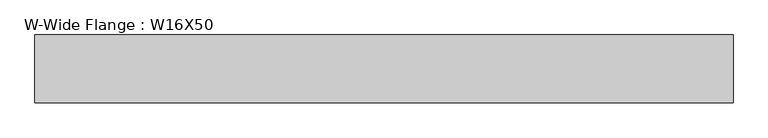
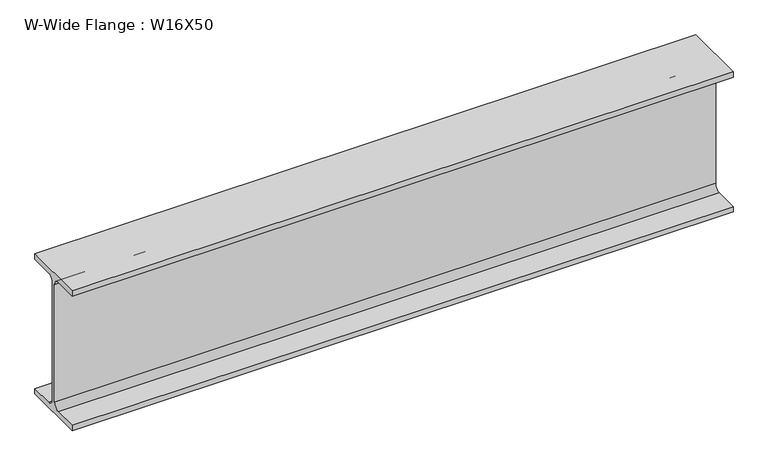
"""IFC4 building model written with IfcOpenShell, lengths in millimetres: beam geometry, W-Wide Flange : W16X50."""

from ifc_helpers import new_model, si_unit, point, frame, frame_2d, origin, place, context, project, spatial, polyline, circle_curve, trimmed, segment, composite_curve, outline, extrude, source, transform, mapped, element, save


def w_wide_flange_w16x50_f430b839(model_context):
    return source(origin(), model_context, "Body", "SweptSolid", [
        extrude(outline(composite_curve([segment(polyline([(-89.789, -191.008), (-22.1615, -191.008)]), True, "CONTINUOUS"), segment(trimmed(circle_curve(frame_2d((-22.1615, -173.6725)), 17.3355), [point((-22.1615, -191.008))], [point((-4.826, -173.6725))], True, "CARTESIAN"), True, "CONTINUOUS"), segment(polyline([(-4.826, -173.6725), (-4.826, 173.6725)]), True, "CONTINUOUS"), segment(trimmed(circle_curve(frame_2d((-22.1615, 173.6725)), 17.3355), [point((-4.826, 173.6725))], [point((-22.1615, 191.008))], True, "CARTESIAN"), True, "CONTINUOUS"), segment(polyline([(-22.1615, 191.008), (-89.789, 191.008), (-89.789, 207.01), (89.789, 207.01), (89.789, 191.008), (22.1615, 191.008)]), True, "CONTINUOUS"), segment(trimmed(circle_curve(frame_2d((22.1615, 173.6725)), 17.3355), [point((22.1615, 191.008))], [point((4.826, 173.6725))], True, "CARTESIAN"), True, "CONTINUOUS"), segment(polyline([(4.826, 173.6725), (4.826, -173.6725)]), True, "CONTINUOUS"), segment(trimmed(circle_curve(frame_2d((22.1615, -173.6725)), 17.3355), [point((4.826, -173.6725))], [point((22.1615, -191.008))], True, "CARTESIAN"), True, "CONTINUOUS"), segment(polyline([(22.1615, -191.008), (89.789, -191.008), (89.789, -207.01), (-89.789, -207.01), (-89.789, -191.008)]), True, "CONTINUOUS")], self_intersect=False)), frame((-912.045346, 0.0, 0.0), z_axis=(1.0, 0.0, 0.0), x_axis=(0.0, 1.0, 0.0)), (0.0, 0.0, 1.0), 1846.950692),
    ])


if __name__ == "__main__":
    model = new_model("IFC4")
    model_context = context("Model", 3, world=origin())
    ifc_project = project(units=[si_unit("LENGTHUNIT", "METRE", prefix="MILLI")], contexts=[model_context])
    site = spatial("IfcSite", under=ifc_project)
    building = spatial("IfcBuilding", under=site)
    placement = place(None, origin())
    w_wide_flange_w16x50_shape = w_wide_flange_w16x50_f430b839(model_context)
    element("IfcBeam", 1, ObjectType="W-Wide Flange : W16X50", at=placement, inside=building, context=model_context, shape_type="MappedRepresentation", body=[
        mapped(w_wide_flange_w16x50_shape, transform((0.0, 0.0, 0.0), x_axis=(1.0, 0.0, 0.0), y_axis=(0.0, 1.0, 0.0), z_axis=(0.0, 0.0, 1.0))),
    ])
    save(model, "model.ifc")

# Revit data of these elements
# Type "W-Wide Flange : W16X50"
#   Assembly Code = "B10"
#   W = 50
#   Start Extension Calculation [instance default] = 10' - 0"
#   Start Extension [instance default] = -0' - 0 1/2"
#   End Extension Calculation [instance default] = 10' - 0"
#   End Extension [instance default] = -0' - 0 1/2"
#   Length [instance default] = 5' - 0"
#   bf = 0' - 7.07"
#   d = 1' - 4.3"
#   k = 0' - 1 5/16"
#   k2 = 0' - 0.6825"
#   tf = 0' - 0.63"
#   tw = 0' - 0.38"
#   A = 0.102083 SF
#   Beam Material [instance default] = Metal - Steel - ASTM A992
# Element 1 (IfcBeam, "W-Wide Flange : W16X50")
#   Materials on its faces: "Metal - Steel - ASTM A992"
# Materials
#   "Metal - Steel - ASTM A992": class "Metal", colour RGB 128 0 0, transparency 0
